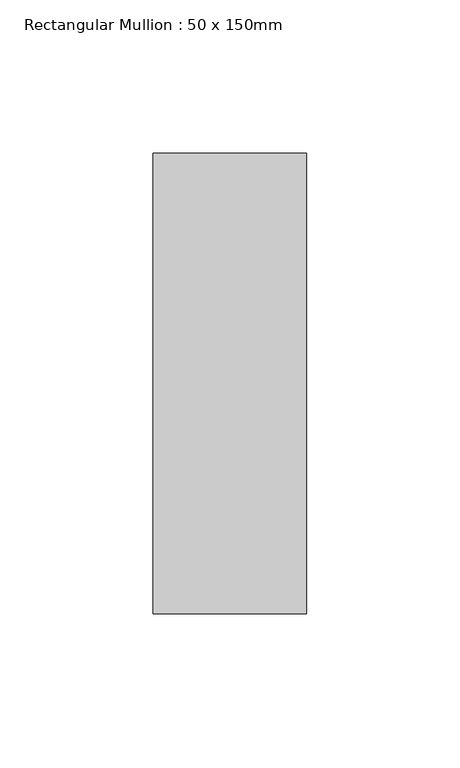
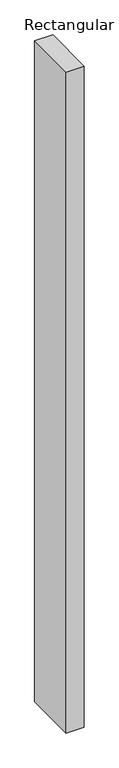
"""IFC4 building model written with IfcOpenShell, lengths in millimetres: member geometry, Rectangular Mullion : 50 x 150mm."""

from ifc_helpers import new_model, si_unit, frame, origin, place, context, project, spatial, polyline, outline, extrude, source, transform, mapped, element, save


def rectangular_mullion_50_x_150mm_d1b252d6(model_context):
    return source(origin(), model_context, "Body", "SweptSolid", [
        extrude(outline(polyline([(0.0, 75.0), (0.0, -75.0), (-50.0, -75.0), (-50.0, 75.0), (0.0, 75.0)])), frame((0.0, 0.0, -1925.0000003), z_axis=(0.0, 0.0, 1.0), x_axis=(1.0, 0.0, 0.0)), (0.0, 0.0, 1.0), 1925.0000003),
    ])


if __name__ == "__main__":
    model = new_model("IFC4")
    model_context = context("Model", 3, world=origin())
    ifc_project = project(units=[si_unit("LENGTHUNIT", "METRE", prefix="MILLI")], contexts=[model_context])
    site = spatial("IfcSite", under=ifc_project)
    building = spatial("IfcBuilding", under=site)
    placement = place(None, origin())
    rectangular_mullion_50_x_150mm_shape = rectangular_mullion_50_x_150mm_d1b252d6(model_context)
    element("IfcMember", 1, ObjectType="Rectangular Mullion : 50 x 150mm", at=placement, inside=building, context=model_context, shape_type="MappedRepresentation", body=[
        mapped(rectangular_mullion_50_x_150mm_shape, transform((0.0, 0.0, 0.0), x_axis=(1.0, 0.0, 0.0), y_axis=(0.0, 1.0, 0.0), z_axis=(0.0, 0.0, 1.0))),
    ])
    save(model, "model.ifc")

# Revit data of these elements
# Type "Rectangular Mullion : 50 x 150mm"
#   built-in parameter 1007304 = 0.492126 (stored number, unit not read)
#   built-in parameter 1007301 = 0.082021 (stored number, unit not read)
#   built-in parameter 1007300 = 0.082021 (stored number, unit not read)
# Element 1 (IfcMember, "Rectangular Mullion : 50 x 150mm")
#   Materials on its faces: "Metal - Aluminium"
# Materials
#   "Metal - Aluminium": class "Metal", colour RGB 247 247 247, transparency 0
